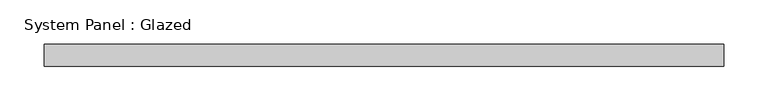
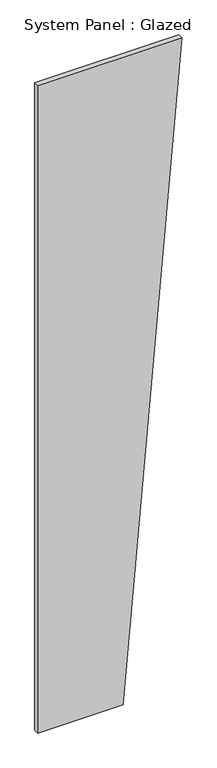
"""IFC4 building model written with IfcOpenShell, lengths in millimetres: plate geometry, System Panel : Glazed."""

from ifc_helpers import new_model, si_unit, frame, origin, place, context, project, spatial, polyline, outline, extrude, source, transform, mapped, element, save


def system_panel_glazed_ca25d662(model_context):
    return source(origin(), model_context, "Body", "SweptSolid", [
        extrude(outline(polyline([(0.0, -386.1685195), (0.0, 71.0314805), (3657.6, 386.1685195), (3657.6, -386.1685195), (0.0, -386.1685195)])), frame((0.0, -44.45, 0.0), z_axis=(0.0, 1.0, 0.0), x_axis=(0.0, 0.0, 1.0)), (0.0, 0.0, 1.0), 25.4),
    ])


if __name__ == "__main__":
    model = new_model("IFC4")
    model_context = context("Model", 3, world=origin())
    ifc_project = project(units=[si_unit("LENGTHUNIT", "METRE", prefix="MILLI")], contexts=[model_context])
    site = spatial("IfcSite", under=ifc_project)
    building = spatial("IfcBuilding", under=site)
    placement = place(None, origin())
    system_panel_glazed_shape = system_panel_glazed_ca25d662(model_context)
    element("IfcPlate", 1, ObjectType="System Panel : Glazed", at=placement, inside=building, context=model_context, shape_type="MappedRepresentation", body=[
        mapped(system_panel_glazed_shape, transform((0.0, 0.0, 0.0), x_axis=(1.0, 0.0, 0.0), y_axis=(0.0, 1.0, 0.0), z_axis=(0.0, 0.0, 1.0))),
    ])
    save(model, "model.ifc")

# Revit data of these elements
# Type "System Panel : Glazed"
#   Construction Type Id = "GSP4R"
#   Analytic Construction = "1/8 in Pilkington single glazing"
#   Visual Light Transmittance = 0.9
#   Solar Heat Gain Coefficient = 0.86
#   Heat Transfer Coefficient (U) = 1.18115 BTU/(h·ft²·°F)
#   Define Thermal Properties by = 1
# Element 1 (IfcPlate, "System Panel : Glazed")
#   Materials on its faces: "Glass"
# Materials
#   "Glass": class "Glass", colour RGB 0 128 192, transparency 0.75, Description = "Soda Lime Glass", Cost = 0
